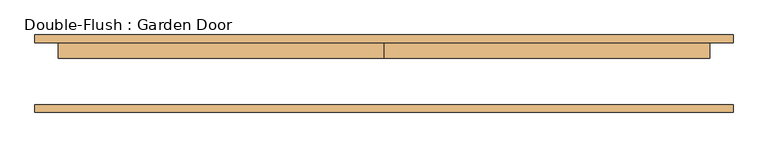
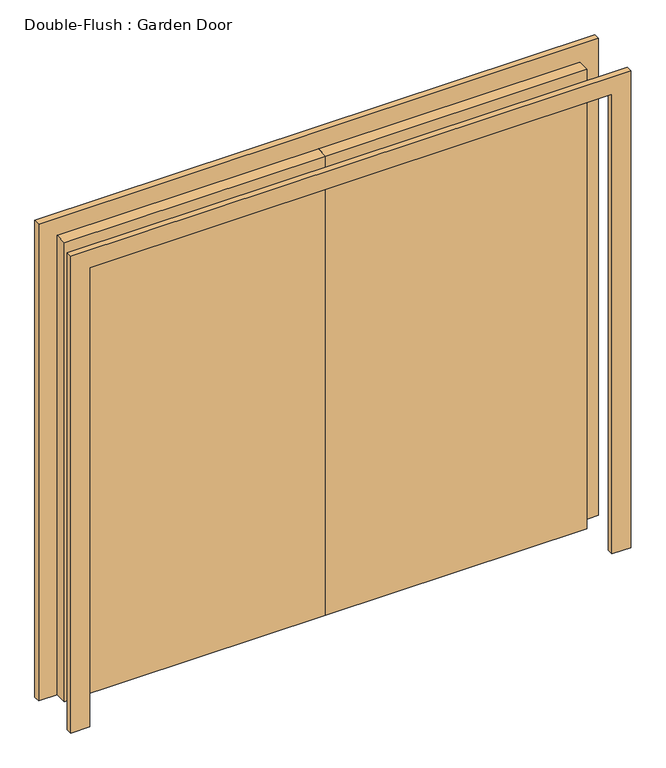
"""IFC4 building model written with IfcOpenShell, lengths in millimetres: door geometry, Double-Flush : Garden Door."""

from ifc_helpers import new_model, si_unit, frame, origin, origin_with_axes, place, context, project, spatial, polyline, outline, extrude, source, transform, mapped, element, save


def double_flush_garden_door_1ae05451(model_context):
    return source(origin(), model_context, "Body", "SweptSolid", [
        extrude(outline(polyline([(0.0, 101.6), (1066.8, 101.6), (1066.8, 50.8), (0.0, 50.8), (0.0, 101.6)])), origin_with_axes(), (0.0, 0.0, 1.0), 1981.2),
        extrude(outline(polyline([(-1066.8, 101.6), (0.0, 101.6), (0.0, 50.8), (-1066.8, 50.8), (-1066.8, 101.6)])), origin_with_axes(), (0.0, 0.0, 1.0), 1981.2),
        extrude(outline(polyline([(1981.2, -1066.8), (1981.2, 1066.8), (0.0, 1066.8), (0.0, 1143.0), (2057.4, 1143.0), (2057.4, -1143.0), (0.0, -1143.0), (0.0, -1066.8), (1981.2, -1066.8)])), frame((0.0, -127.0, 0.0), z_axis=(0.0, 1.0, 0.0), x_axis=(0.0, 0.0, 1.0)), (0.0, 0.0, 1.0), 25.4),
        extrude(outline(polyline([(1981.2, -1066.8), (1981.2, 1066.8), (0.0, 1066.8), (0.0, 1143.0), (2057.4, 1143.0), (2057.4, -1143.0), (0.0, -1143.0), (0.0, -1066.8), (1981.2, -1066.8)])), frame((0.0, 101.6, 0.0), z_axis=(0.0, 1.0, 0.0), x_axis=(0.0, 0.0, 1.0)), (0.0, 0.0, 1.0), 25.4),
    ])


if __name__ == "__main__":
    model = new_model("IFC4")
    model_context = context("Model", 3, world=origin())
    ifc_project = project(units=[si_unit("LENGTHUNIT", "METRE", prefix="MILLI")], contexts=[model_context])
    site = spatial("IfcSite", under=ifc_project)
    building = spatial("IfcBuilding", under=site)
    placement = place(None, origin())
    double_flush_garden_door_shape = double_flush_garden_door_1ae05451(model_context)
    element("IfcDoor", 1, ObjectType="Double-Flush : Garden Door", at=placement, inside=building, context=model_context, shape_type="MappedRepresentation", body=[
        mapped(double_flush_garden_door_shape, transform((0.0, 0.0, 0.0), x_axis=(1.0, 0.0, 0.0), y_axis=(0.0, 1.0, 0.0), z_axis=(0.0, 0.0, 1.0))),
    ])
    save(model, "model.ifc")

# Revit data of these elements
# Type "Double-Flush : Garden Door"
#   Type Mark = "23"
#   Assembly Code = "C1020"
#   Thickness = 0' - 2"
#   Height = 6' - 6"
#   Trim Projection Ext = 0' - 1"
#   Trim Projection Int = 0' - 1"
#   Trim Width = 0' - 3"
#   Width = 7' - 0"
#   Function = 0
#   Door Material = Default
#   Frame Material = Door - Panel
#   Wall Closure = (empty or 0)
# Element 1 (IfcDoor, "Double-Flush : Garden Door")
#   Materials on its faces: "Door - Panel", "Default"
# Materials
#   "Default": class "Unassigned", colour RGB 127 127 127, transparency 0, Comments = "Rendering appearance not upgraded Rendering appearance not upgraded "
#   "Door - Panel": class "Wood", colour RGB 149 143 132, transparency 0, Comments = "Rendering appearance not upgraded Rendering appearance not upgraded "
